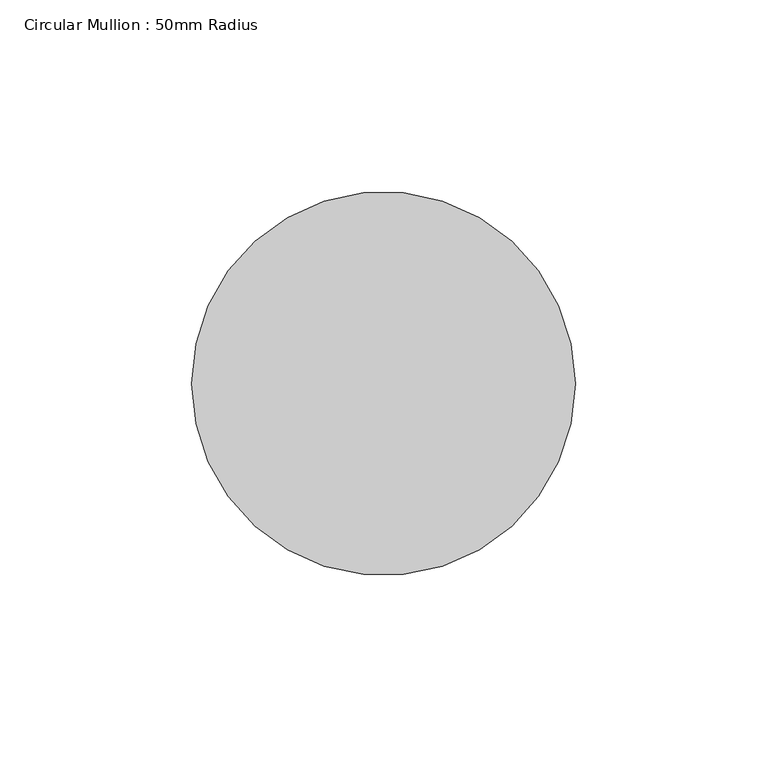
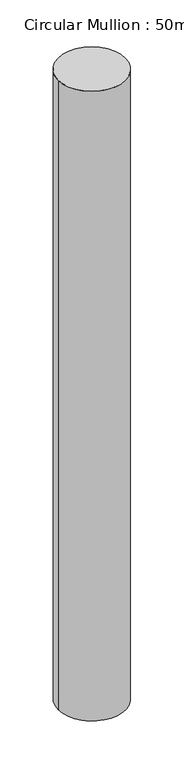
"""IFC4 building model written with IfcOpenShell, lengths in millimetres: member geometry, Circular Mullion : 50mm Radius."""

from ifc_helpers import new_model, si_unit, point, frame, origin, origin_2d, place, context, project, spatial, circle_curve, trimmed, segment, composite_curve, outline, extrude, source, transform, mapped, element, save


def circular_mullion_50mm_radius_4de79c80(model_context):
    return source(origin(), model_context, "Body", "SweptSolid", [
        extrude(outline(composite_curve([segment(trimmed(circle_curve(origin_2d(), 50.0), [point((50.0, 0.0))], [point((-50.0, 0.0))], False, "CARTESIAN"), True, "CONTINUOUS"), segment(trimmed(circle_curve(origin_2d(), 50.0), [point((-50.0, 0.0))], [point((50.0, 0.0))], False, "CARTESIAN"), True, "CONTINUOUS")], self_intersect=False)), frame((0.0, 0.0, -991.0264025), z_axis=(0.0, 0.0, 1.0), x_axis=(1.0, 0.0, 0.0)), (0.0, 0.0, 1.0), 991.0264025),
    ])


if __name__ == "__main__":
    model = new_model("IFC4")
    model_context = context("Model", 3, world=origin())
    ifc_project = project(units=[si_unit("LENGTHUNIT", "METRE", prefix="MILLI")], contexts=[model_context])
    site = spatial("IfcSite", under=ifc_project)
    building = spatial("IfcBuilding", under=site)
    placement = place(None, origin())
    circular_mullion_50mm_radius_shape = circular_mullion_50mm_radius_4de79c80(model_context)
    element("IfcMember", 1, ObjectType="Circular Mullion : 50mm Radius", at=placement, inside=building, context=model_context, shape_type="MappedRepresentation", body=[
        mapped(circular_mullion_50mm_radius_shape, transform((0.0, 0.0, 0.0), x_axis=(1.0, 0.0, 0.0), y_axis=(0.0, 1.0, 0.0), z_axis=(0.0, 0.0, 1.0))),
    ])
    save(model, "model.ifc")

# Revit data of these elements
# Type "Circular Mullion : 50mm Radius"
#   built-in parameter 1007350 = 0.164042 (stored number, unit not read)
# Element 1 (IfcMember, "Circular Mullion : 50mm Radius")
#   Materials on its faces: "Aluminium"
# Materials
#   "Aluminium": class "Metal", colour RGB 247 247 247, transparency 0, Description = "Aluminium 6061", Cost = 0
